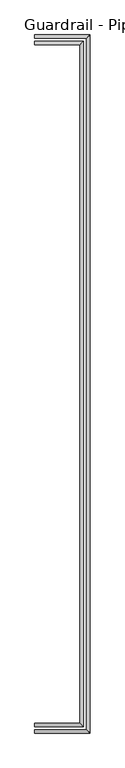
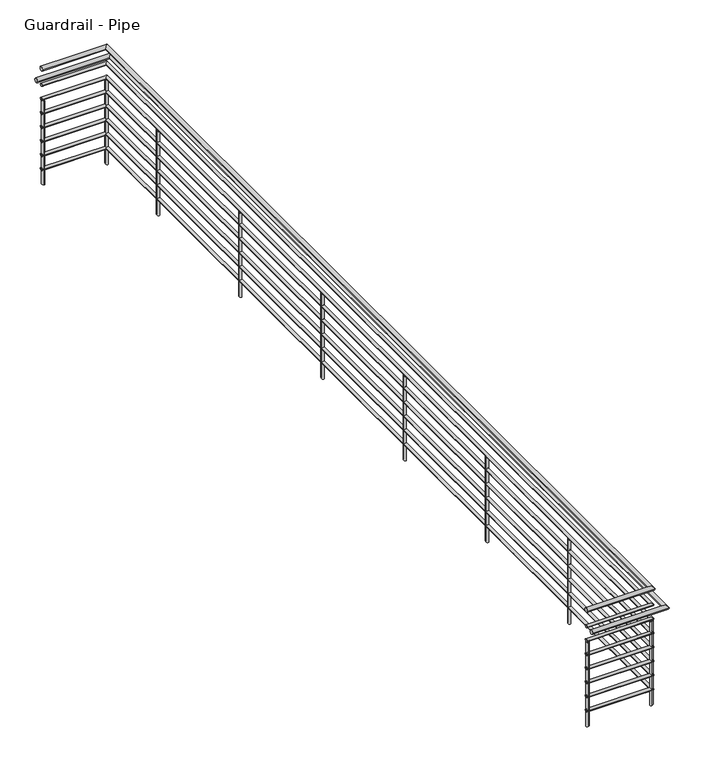
"""IFC4 building model written with IfcOpenShell, lengths in millimetres: railing geometry, Guardrail - Pipe."""

import ifcopenshell
import ifcopenshell.guid

model = None  # the IFC model being written
_history = None  # IfcOwnerHistory: only IFC2X3 demands one
_inside = {}  # id of a spatial element -> (the spatial element, [elements in it])
_under = {}  # id of a project, library or spatial element -> (it, [spatial elements below it])
_declared = {}  # id of a project -> (the project, [libraries it declares])
_typed = {}  # id of a type object -> (the type object, [elements of that type])
_made_of = {}  # id of a material, layer set ... -> (it, [elements and type objects made of it])


def new_model(schema):
    """Start an empty IFC model of exactly this schema.

    Asked for "IFC4X3", IfcOpenShell would pick the latest addendum, in which some entities
    have other attributes; the version numbers below select the first issue.
    IFC2X3 requires an IfcOwnerHistory on every rooted entity: one is made here for all.
    """
    global model, _history
    if schema == "IFC4X3":
        model = ifcopenshell.file(schema_version=(4, 3, 0, 0))
    else:
        model = ifcopenshell.file(schema=schema)
    _inside.clear()
    _under.clear()
    _declared.clear()
    _typed.clear()
    _made_of.clear()
    _history = None
    if model.schema == "IFC2X3":
        org = make("IfcOrganization", Name="unknown")
        user = make(
            "IfcPersonAndOrganization",
            ThePerson=make("IfcPerson", FamilyName="unknown"),
            TheOrganization=org,
        )
        app = make(
            "IfcApplication",
            ApplicationDeveloper=org,
            Version="unknown",
            ApplicationFullName="unknown",
            ApplicationIdentifier="unknown",
        )
        _history = make(
            "IfcOwnerHistory",
            OwningUser=user,
            OwningApplication=app,
            ChangeAction="ADDED",
            CreationDate=0,
        )
    return model


def make(cls, **values):
    """One entity of the class cls with the attributes given. An attribute that is None is left unset."""
    return model.create_entity(
        cls, **{name: value for name, value in values.items() if value is not None}
    )


def rooted(cls, **values):
    """An entity with a GlobalId (a new one), such as an element, a storey or a relation."""
    return make(cls, GlobalId=ifcopenshell.guid.new(), OwnerHistory=_history, **values)


def si_unit(unit_type, name, prefix=None):
    """IfcSIUnit, for example si_unit("LENGTHUNIT", "METRE", prefix="MILLI")."""
    return make("IfcSIUnit", UnitType=unit_type, Prefix=prefix, Name=name)


def assignment(units):
    """IfcUnitAssignment: the units of a project."""
    return None if units is None else make("IfcUnitAssignment", Units=units)


def point(xyz):
    """IfcCartesianPoint."""
    return None if xyz is None else make("IfcCartesianPoint", Coordinates=xyz)


def direction(xyz):
    """IfcDirection."""
    return None if xyz is None else make("IfcDirection", DirectionRatios=xyz)


def frame(location, z_axis=None, x_axis=None):
    """IfcAxis2Placement3D, a coordinate frame: its origin and axes. An axis left out is left unset."""
    return make(
        "IfcAxis2Placement3D",
        Location=point(location),
        Axis=direction(z_axis),
        RefDirection=direction(x_axis),
    )


def origin():
    """The frame at (0, 0, 0) with its axes left unset."""
    return frame((0.0, 0.0, 0.0))


def place(relative_to, where):
    """IfcLocalPlacement: puts the frame where relative to a parent placement (None: the world)."""
    return make(
        "IfcLocalPlacement", PlacementRelTo=relative_to, RelativePlacement=where
    )


def context(
    kind, dimensions, precision=None, world=None, true_north=None, identifier=None
):
    """IfcGeometricRepresentationContext, for example the 3D "Model" context."""
    return make(
        "IfcGeometricRepresentationContext",
        ContextIdentifier=identifier,
        ContextType=kind,
        CoordinateSpaceDimension=dimensions,
        Precision=precision,
        WorldCoordinateSystem=world,
        TrueNorth=true_north,
    )


def project(units=None, contexts=None):
    """IfcProject with its units and contexts."""
    return rooted(
        "IfcProject",
        Name="project",
        RepresentationContexts=contexts,
        UnitsInContext=assignment(units),
    )


def spatial(cls, under=None, at=None, **own):
    """A site, building, storey or space (cls), placed at a placement, below another one or the project."""
    s = rooted(cls, ObjectPlacement=at, **own)
    if under is not None:
        _under.setdefault(under.id(), (under, []))[1].append(s)
    return s


def circle_curve(where, radius):
    """IfcCircle in the frame where."""
    return make("IfcCircle", Position=where, Radius=radius)


def ellipse_curve(where, semi_axis1, semi_axis2):
    """IfcEllipse in the frame where."""
    return make(
        "IfcEllipse", Position=where, SemiAxis1=semi_axis1, SemiAxis2=semi_axis2
    )


def shape(context_of_items, identifier, shape_type, items):
    """IfcShapeRepresentation: the items that make up one representation, for example the "Body"."""
    return make(
        "IfcShapeRepresentation",
        ContextOfItems=context_of_items,
        RepresentationIdentifier=identifier,
        RepresentationType=shape_type,
        Items=items,
    )


def source(mapping_origin, context_of_items, identifier, shape_type, items):
    """IfcRepresentationMap: a shape defined once, which mapped items show again and again."""
    return make(
        "IfcRepresentationMap",
        MappingOrigin=mapping_origin,
        MappedRepresentation=shape(context_of_items, identifier, shape_type, items),
    )


def transform(
    local_origin,
    x_axis=None,
    y_axis=None,
    z_axis=None,
    scale=None,
    scale2=None,
    scale3=None,
    uniform=True,
):
    """IfcCartesianTransformationOperator3D, or its non-uniform kind. x_axis, y_axis, z_axis: its Axis1, 2, 3."""
    if uniform:
        return make(
            "IfcCartesianTransformationOperator3D",
            Axis1=direction(x_axis),
            Axis2=direction(y_axis),
            LocalOrigin=point(local_origin),
            Scale=scale,
            Axis3=direction(z_axis),
        )
    return make(
        "IfcCartesianTransformationOperator3DnonUniform",
        Axis1=direction(x_axis),
        Axis2=direction(y_axis),
        LocalOrigin=point(local_origin),
        Scale=scale,
        Axis3=direction(z_axis),
        Scale2=scale2,
        Scale3=scale3,
    )


def mapped(mapping_source, mapping_target):
    """IfcMappedItem: shows the shape of a source again, moved by a transform."""
    return make(
        "IfcMappedItem", MappingSource=mapping_source, MappingTarget=mapping_target
    )


def made_of(thing, what):
    """Note that an element or type object is made of a material, layer set ...; save() writes the relation."""
    if what is not None:
        _made_of.setdefault(what.id(), (what, []))[1].append(thing)
    return thing


def element(
    cls,
    number,
    at=None,
    inside=None,
    cuts=None,
    type_object=None,
    material=None,
    context=None,
    identifier="Body",
    shape_type=None,
    held_by="IfcProductDefinitionShape",
    body=None,
    shapes=None,
    **own,
):
    """One element of the class cls, such as IfcWall. Its Tag is "e" and its number.

    at: its placement. inside: the storey or other place that contains it. cuts: it is an
    opening in that element (IfcRelVoidsElement). A single representation is given by context,
    identifier, shape_type and body (its items); several are given by shapes. held_by: the class
    of the entity that holds the representations. save() writes the other relations.
    """
    e = rooted(cls, Tag="e%d" % number, ObjectPlacement=at, **own)
    if body is not None:
        shapes = [shape(context, identifier, shape_type, body)]
    if shapes is not None:
        e.Representation = make(held_by, Representations=shapes)
    if inside is not None:
        _inside.setdefault(inside.id(), (inside, []))[1].append(e)
    if cuts is not None:
        rooted(
            "IfcRelVoidsElement", RelatingBuildingElement=cuts, RelatedOpeningElement=e
        )
    if type_object is not None:
        _typed.setdefault(type_object.id(), (type_object, []))[1].append(e)
    return made_of(e, material)


def aggregate(whole, parts):
    """IfcRelAggregates: a whole, such as a stair, and the parts it consists of."""
    return rooted("IfcRelAggregates", RelatingObject=whole, RelatedObjects=parts)


def save(model, path):
    """Write the relations noted so far, then the file.

    IfcRelAggregates (storeys below a building ...), IfcRelContainedInSpatialStructure (elements
    in a storey), IfcRelDefinesByType, IfcRelAssociatesMaterial and IfcRelDeclares: one each for
    every whole, place, type object, material and project.
    """
    for whole, parts in _under.values():
        aggregate(whole, parts)
    for where, things in _inside.values():
        rooted(
            "IfcRelContainedInSpatialStructure",
            RelatedElements=things,
            RelatingStructure=where,
        )
    for kind, things in _typed.values():
        rooted("IfcRelDefinesByType", RelatedObjects=things, RelatingType=kind)
    for what, things in _made_of.values():
        rooted("IfcRelAssociatesMaterial", RelatedObjects=things, RelatingMaterial=what)
    for by, libraries in _declared.values():
        rooted("IfcRelDeclares", RelatingContext=by, RelatedDefinitions=libraries)
    model.write(path)


def plane_surface(at):
    """IfcPlane: the flat surface through the origin of the frame at, square to its z axis."""
    return make("IfcPlane", Position=at)


def cylinder_surface(at, radius):
    """IfcCylindricalSurface: all points at the distance radius from the z axis of the frame at."""
    return make("IfcCylindricalSurface", Position=at, Radius=radius)


def advanced_brep(points, edges, surfaces, faces):
    """IfcAdvancedBrep: a solid bounded by faces that lie on surfaces and meet in shared edges.

    An edge is (start, end): straight between two places in points (the first is 0);
    or (start, end, curve); or (start, end, curve, False) where it runs against its curve.
    A face is (place in surfaces, loops), or (place, loops, False) where it looks against
    its surface's normal. A loop lists edges by number (the first is 1), with a minus sign
    where the edge is run from its end to its start. The first loop is the outer one.
    """
    corners = [point(p) for p in points]
    vertices = [make("IfcVertexPoint", VertexGeometry=c) for c in corners]
    made = []
    for start, end, *more in edges:
        made.append(
            make(
                "IfcEdgeCurve",
                EdgeStart=vertices[start],
                EdgeEnd=vertices[end],
                EdgeGeometry=more[0] if more else make("IfcPolyline", Points=[corners[start], corners[end]]),
                SameSense=more[1] if len(more) > 1 else True,
            )
        )
    hull = []
    for where, loops, *sense in faces:
        bounds = []
        for j, loop in enumerate(loops):
            ring = [make("IfcOrientedEdge", EdgeElement=made[abs(k) - 1], Orientation=k > 0) for k in loop]
            bounds.append(
                make(
                    "IfcFaceOuterBound" if j == 0 else "IfcFaceBound",
                    Bound=make("IfcEdgeLoop", EdgeList=ring),
                    Orientation=True,
                )
            )
        hull.append(make("IfcAdvancedFace", Bounds=bounds, FaceSurface=surfaces[where], SameSense=sense[0] if sense else True))
    return make("IfcAdvancedBrep", Outer=make("IfcClosedShell", CfsFaces=hull))


def guardrail_pipe_ba8d120a(model_context):
    return source(origin(), model_context, "Body", "AdvancedBrep", [
        advanced_brep(
        [(13389.3313551, 10867.95, 4705.35), (13389.3313551, 10906.05, 4705.35), (13967.1813551, 10867.95, 4705.35), (13929.0813551, 10906.05, 4705.35), (13967.1813551, 18983.25, 4705.35), (13929.0813551, 18945.15, 4705.35), (13389.3313551, 18983.25, 4705.35), (13389.3313551, 18945.15, 4705.35)],
        [
            (0, 1, circle_curve(frame((13389.3313551, 10887.0, 4705.35), z_axis=(-1.0, 0.0, 0.0), x_axis=(0.0, 1.0, 0.0)), 19.05)),
            (1, 0, circle_curve(frame((13389.3313551, 10887.0, 4705.35), z_axis=(-1.0, 0.0, 0.0), x_axis=(0.0, 1.0, 0.0)), 19.05)),
            (0, 2),
            (2, 3, ellipse_curve(frame((13948.1313551, 10887.0, 4705.35), z_axis=(-0.7071067811865475, -0.7071067811865475, 0.0), x_axis=(-0.7071067811865476, 0.7071067811865474, 0.0)), 26.9407684, 19.05)),
            (3, 1),
            (3, 2, ellipse_curve(frame((13948.1313551, 10887.0, 4705.35), z_axis=(-0.7071067811865475, -0.7071067811865475, 0.0), x_axis=(-0.7071067811865476, 0.7071067811865474, 0.0)), 26.9407684, 19.05)),
            (2, 4),
            (4, 5, ellipse_curve(frame((13948.1313551, 18964.2, 4705.35), z_axis=(0.7071067811865475, -0.7071067811865475, 0.0), x_axis=(-0.7071067811865474, -0.7071067811865476, 0.0)), 26.9407684, 19.05)),
            (5, 3),
            (5, 4, ellipse_curve(frame((13948.1313551, 18964.2, 4705.35), z_axis=(0.7071067811865475, -0.7071067811865475, 0.0), x_axis=(-0.7071067811865474, -0.7071067811865476, 0.0)), 26.9407684, 19.05)),
            (6, 7, circle_curve(frame((13389.3313551, 18964.2, 4705.35), z_axis=(-1.0, 0.0, 0.0), x_axis=(0.0, -1.0, 0.0)), 19.05)),
            (7, 6, circle_curve(frame((13389.3313551, 18964.2, 4705.35), z_axis=(-1.0, 0.0, 0.0), x_axis=(0.0, -1.0, 0.0)), 19.05)),
            (4, 6),
            (7, 5),
        ],
        [
            plane_surface(frame((13389.3313551, 10887.0, 4724.4), z_axis=(-1.0, 0.0, 0.0), x_axis=(0.0, 1.0, 0.0))),
            cylinder_surface(frame((13389.3313551, 10887.0, 4705.35), z_axis=(-1.0, 0.0, 0.0), x_axis=(0.0, 1.0, 0.0)), 19.05),
            cylinder_surface(frame((13948.1313551, 10887.0, 4705.35), z_axis=(0.0, -1.0, 0.0), x_axis=(-1.0, 0.0, 0.0)), 19.05),
            plane_surface(frame((13389.3313551, 18964.2, 4724.4), z_axis=(-1.0, 0.0, 0.0), x_axis=(0.0, -1.0, 0.0))),
            cylinder_surface(frame((13948.1313551, 18964.2, 4705.35), z_axis=(1.0, 0.0, 0.0), x_axis=(0.0, -1.0, 0.0)), 19.05),
        ],
        [
            (0, [[1, 2]]),
            (1, [[-1, 3, 4, 5]]),
            (1, [[-2, -5, 6, -3]]),
            (2, [[-4, 7, 8, 9]]),
            (2, [[-6, -9, 10, -7]]),
            (3, [[11, 12]]),
            (4, [[-8, 13, -12, 14]]),
            (4, [[-10, -14, -11, -13]]),
        ],
    ),
        advanced_brep(
        [(13389.3313551, 10874.3, 4559.3), (13389.3313551, 10899.7, 4559.3), (13960.8313551, 10874.3, 4559.3), (13935.4313551, 10899.7, 4559.3), (13960.8313551, 18976.9, 4559.3), (13935.4313551, 18951.5, 4559.3), (13389.3313551, 18976.9, 4559.3), (13389.3313551, 18951.5, 4559.3)],
        [
            (0, 1, circle_curve(frame((13389.3313551, 10887.0, 4559.3), z_axis=(-1.0, 0.0, 0.0), x_axis=(0.0, 1.0, 0.0)), 12.7)),
            (1, 0, circle_curve(frame((13389.3313551, 10887.0, 4559.3), z_axis=(-1.0, 0.0, 0.0), x_axis=(0.0, 1.0, 0.0)), 12.7)),
            (0, 2),
            (2, 3, ellipse_curve(frame((13948.1313551, 10887.0, 4559.3), z_axis=(-0.7071067811865475, -0.7071067811865475, 0.0), x_axis=(-0.7071067811865476, 0.7071067811865474, 0.0)), 17.9605122, 12.7)),
            (3, 1),
            (3, 2, ellipse_curve(frame((13948.1313551, 10887.0, 4559.3), z_axis=(-0.7071067811865475, -0.7071067811865475, 0.0), x_axis=(-0.7071067811865476, 0.7071067811865474, 0.0)), 17.9605122, 12.7)),
            (2, 4),
            (4, 5, ellipse_curve(frame((13948.1313551, 18964.2, 4559.3), z_axis=(0.7071067811865475, -0.7071067811865475, 0.0), x_axis=(-0.7071067811865474, -0.7071067811865476, 0.0)), 17.9605122, 12.7)),
            (5, 3),
            (5, 4, ellipse_curve(frame((13948.1313551, 18964.2, 4559.3), z_axis=(0.7071067811865475, -0.7071067811865475, 0.0), x_axis=(-0.7071067811865474, -0.7071067811865476, 0.0)), 17.9605122, 12.7)),
            (6, 7, circle_curve(frame((13389.3313551, 18964.2, 4559.3), z_axis=(-1.0, 0.0, 0.0), x_axis=(0.0, -1.0, 0.0)), 12.7)),
            (7, 6, circle_curve(frame((13389.3313551, 18964.2, 4559.3), z_axis=(-1.0, 0.0, 0.0), x_axis=(0.0, -1.0, 0.0)), 12.7)),
            (4, 6),
            (7, 5),
        ],
        [
            plane_surface(frame((13389.3313551, 10887.0, 4572.0), z_axis=(-1.0, 0.0, 0.0), x_axis=(0.0, 1.0, 0.0))),
            cylinder_surface(frame((13389.3313551, 10887.0, 4559.3), z_axis=(-1.0, 0.0, 0.0), x_axis=(0.0, 1.0, 0.0)), 12.7),
            cylinder_surface(frame((13948.1313551, 10887.0, 4559.3), z_axis=(0.0, -1.0, 0.0), x_axis=(-1.0, 0.0, 0.0)), 12.7),
            plane_surface(frame((13389.3313551, 18964.2, 4572.0), z_axis=(-1.0, 0.0, 0.0), x_axis=(0.0, -1.0, 0.0))),
            cylinder_surface(frame((13948.1313551, 18964.2, 4559.3), z_axis=(1.0, 0.0, 0.0), x_axis=(0.0, -1.0, 0.0)), 12.7),
        ],
        [
            (0, [[1, 2]]),
            (1, [[-1, 3, 4, 5]]),
            (1, [[-2, -5, 6, -3]]),
            (2, [[-4, 7, 8, 9]]),
            (2, [[-6, -9, 10, -7]]),
            (3, [[11, 12]]),
            (4, [[-8, 13, -12, 14]]),
            (4, [[-10, -14, -11, -13]]),
        ],
    ),
        advanced_brep(
        [(13389.3313551, 10791.75, 4552.95), (13389.3313551, 10829.85, 4552.95), (14043.3813551, 10791.75, 4552.95), (14005.2813551, 10829.85, 4552.95), (14043.3813551, 19059.45, 4552.95), (14005.2813551, 19021.35, 4552.95), (13389.3313551, 19059.45, 4552.95), (13389.3313551, 19021.35, 4552.95)],
        [
            (0, 1, circle_curve(frame((13389.3313551, 10810.8, 4552.95), z_axis=(-1.0, 0.0, 0.0), x_axis=(0.0, 1.0, 0.0)), 19.05)),
            (1, 0, circle_curve(frame((13389.3313551, 10810.8, 4552.95), z_axis=(-1.0, 0.0, 0.0), x_axis=(0.0, 1.0, 0.0)), 19.05)),
            (0, 2),
            (2, 3, ellipse_curve(frame((14024.3313551, 10810.8, 4552.95), z_axis=(-0.7071067811865475, -0.7071067811865475, 0.0), x_axis=(-0.7071067811865476, 0.7071067811865474, 0.0)), 26.9407684, 19.05)),
            (3, 1),
            (3, 2, ellipse_curve(frame((14024.3313551, 10810.8, 4552.95), z_axis=(-0.7071067811865475, -0.7071067811865475, 0.0), x_axis=(-0.7071067811865476, 0.7071067811865474, 0.0)), 26.9407684, 19.05)),
            (2, 4),
            (4, 5, ellipse_curve(frame((14024.3313551, 19040.4, 4552.95), z_axis=(0.7071067811865475, -0.7071067811865475, 0.0), x_axis=(-0.7071067811865474, -0.7071067811865476, 0.0)), 26.9407684, 19.05)),
            (5, 3),
            (5, 4, ellipse_curve(frame((14024.3313551, 19040.4, 4552.95), z_axis=(0.7071067811865475, -0.7071067811865475, 0.0), x_axis=(-0.7071067811865474, -0.7071067811865476, 0.0)), 26.9407684, 19.05)),
            (6, 7, circle_curve(frame((13389.3313551, 19040.4, 4552.95), z_axis=(-1.0, 0.0, 0.0), x_axis=(0.0, -1.0, 0.0)), 19.05)),
            (7, 6, circle_curve(frame((13389.3313551, 19040.4, 4552.95), z_axis=(-1.0, 0.0, 0.0), x_axis=(0.0, -1.0, 0.0)), 19.05)),
            (4, 6),
            (7, 5),
        ],
        [
            plane_surface(frame((13389.3313551, 10810.8, 4572.0), z_axis=(-1.0, 0.0, 0.0), x_axis=(0.0, 1.0, 0.0))),
            cylinder_surface(frame((13389.3313551, 10810.8, 4552.95), z_axis=(-1.0, 0.0, 0.0), x_axis=(0.0, 1.0, 0.0)), 19.05),
            cylinder_surface(frame((14024.3313551, 10810.8, 4552.95), z_axis=(0.0, -1.0, 0.0), x_axis=(-1.0, 0.0, 0.0)), 19.05),
            plane_surface(frame((13389.3313551, 19040.4, 4572.0), z_axis=(-1.0, 0.0, 0.0), x_axis=(0.0, -1.0, 0.0))),
            cylinder_surface(frame((14024.3313551, 19040.4, 4552.95), z_axis=(1.0, 0.0, 0.0), x_axis=(0.0, -1.0, 0.0)), 19.05),
        ],
        [
            (0, [[1, 2]]),
            (1, [[-1, 3, 4, 5]]),
            (1, [[-2, -5, 6, -3]]),
            (2, [[-4, 7, 8, 9]]),
            (2, [[-6, -9, 10, -7]]),
            (3, [[11, 12]]),
            (4, [[-8, 13, -12, 14]]),
            (4, [[-10, -14, -11, -13]]),
        ],
    ),
        advanced_brep(
        [(13389.3313551, 10874.3, 4432.3), (13389.3313551, 10899.7, 4432.3), (13960.8313551, 10874.3, 4432.3), (13935.4313551, 10899.7, 4432.3), (13960.8313551, 18976.9, 4432.3), (13935.4313551, 18951.5, 4432.3), (13389.3313551, 18976.9, 4432.3), (13389.3313551, 18951.5, 4432.3)],
        [
            (0, 1, circle_curve(frame((13389.3313551, 10887.0, 4432.3), z_axis=(-1.0, 0.0, 0.0), x_axis=(0.0, 1.0, 0.0)), 12.7)),
            (1, 0, circle_curve(frame((13389.3313551, 10887.0, 4432.3), z_axis=(-1.0, 0.0, 0.0), x_axis=(0.0, 1.0, 0.0)), 12.7)),
            (0, 2),
            (2, 3, ellipse_curve(frame((13948.1313551, 10887.0, 4432.3), z_axis=(-0.7071067811865475, -0.7071067811865475, 0.0), x_axis=(-0.7071067811865476, 0.7071067811865474, 0.0)), 17.9605122, 12.7)),
            (3, 1),
            (3, 2, ellipse_curve(frame((13948.1313551, 10887.0, 4432.3), z_axis=(-0.7071067811865475, -0.7071067811865475, 0.0), x_axis=(-0.7071067811865476, 0.7071067811865474, 0.0)), 17.9605122, 12.7)),
            (2, 4),
            (4, 5, ellipse_curve(frame((13948.1313551, 18964.2, 4432.3), z_axis=(0.7071067811865475, -0.7071067811865475, 0.0), x_axis=(-0.7071067811865474, -0.7071067811865476, 0.0)), 17.9605122, 12.7)),
            (5, 3),
            (5, 4, ellipse_curve(frame((13948.1313551, 18964.2, 4432.3), z_axis=(0.7071067811865475, -0.7071067811865475, 0.0), x_axis=(-0.7071067811865474, -0.7071067811865476, 0.0)), 17.9605122, 12.7)),
            (6, 7, circle_curve(frame((13389.3313551, 18964.2, 4432.3), z_axis=(-1.0, 0.0, 0.0), x_axis=(0.0, -1.0, 0.0)), 12.7)),
            (7, 6, circle_curve(frame((13389.3313551, 18964.2, 4432.3), z_axis=(-1.0, 0.0, 0.0), x_axis=(0.0, -1.0, 0.0)), 12.7)),
            (4, 6),
            (7, 5),
        ],
        [
            plane_surface(frame((13389.3313551, 10887.0, 4445.0), z_axis=(-1.0, 0.0, 0.0), x_axis=(0.0, 1.0, 0.0))),
            cylinder_surface(frame((13389.3313551, 10887.0, 4432.3), z_axis=(-1.0, 0.0, 0.0), x_axis=(0.0, 1.0, 0.0)), 12.7),
            cylinder_surface(frame((13948.1313551, 10887.0, 4432.3), z_axis=(0.0, -1.0, 0.0), x_axis=(-1.0, 0.0, 0.0)), 12.7),
            plane_surface(frame((13389.3313551, 18964.2, 4445.0), z_axis=(-1.0, 0.0, 0.0), x_axis=(0.0, -1.0, 0.0))),
            cylinder_surface(frame((13948.1313551, 18964.2, 4432.3), z_axis=(1.0, 0.0, 0.0), x_axis=(0.0, -1.0, 0.0)), 12.7),
        ],
        [
            (0, [[1, 2]]),
            (1, [[-1, 3, 4, 5]]),
            (1, [[-2, -5, 6, -3]]),
            (2, [[-4, 7, 8, 9]]),
            (2, [[-6, -9, 10, -7]]),
            (3, [[11, 12]]),
            (4, [[-8, 13, -12, 14]]),
            (4, [[-10, -14, -11, -13]]),
        ],
    ),
        advanced_brep(
        [(13389.3313551, 10874.3, 4305.3), (13389.3313551, 10899.7, 4305.3), (13960.8313551, 10874.3, 4305.3), (13935.4313551, 10899.7, 4305.3), (13960.8313551, 18976.9, 4305.3), (13935.4313551, 18951.5, 4305.3), (13389.3313551, 18976.9, 4305.3), (13389.3313551, 18951.5, 4305.3)],
        [
            (0, 1, circle_curve(frame((13389.3313551, 10887.0, 4305.3), z_axis=(-1.0, 0.0, 0.0), x_axis=(0.0, 1.0, 0.0)), 12.7)),
            (1, 0, circle_curve(frame((13389.3313551, 10887.0, 4305.3), z_axis=(-1.0, 0.0, 0.0), x_axis=(0.0, 1.0, 0.0)), 12.7)),
            (0, 2),
            (2, 3, ellipse_curve(frame((13948.1313551, 10887.0, 4305.3), z_axis=(-0.7071067811865475, -0.7071067811865475, 0.0), x_axis=(-0.7071067811865476, 0.7071067811865474, 0.0)), 17.9605122, 12.7)),
            (3, 1),
            (3, 2, ellipse_curve(frame((13948.1313551, 10887.0, 4305.3), z_axis=(-0.7071067811865475, -0.7071067811865475, 0.0), x_axis=(-0.7071067811865476, 0.7071067811865474, 0.0)), 17.9605122, 12.7)),
            (2, 4),
            (4, 5, ellipse_curve(frame((13948.1313551, 18964.2, 4305.3), z_axis=(0.7071067811865475, -0.7071067811865475, 0.0), x_axis=(-0.7071067811865474, -0.7071067811865476, 0.0)), 17.9605122, 12.7)),
            (5, 3),
            (5, 4, ellipse_curve(frame((13948.1313551, 18964.2, 4305.3), z_axis=(0.7071067811865475, -0.7071067811865475, 0.0), x_axis=(-0.7071067811865474, -0.7071067811865476, 0.0)), 17.9605122, 12.7)),
            (6, 7, circle_curve(frame((13389.3313551, 18964.2, 4305.3), z_axis=(-1.0, 0.0, 0.0), x_axis=(0.0, -1.0, 0.0)), 12.7)),
            (7, 6, circle_curve(frame((13389.3313551, 18964.2, 4305.3), z_axis=(-1.0, 0.0, 0.0), x_axis=(0.0, -1.0, 0.0)), 12.7)),
            (4, 6),
            (7, 5),
        ],
        [
            plane_surface(frame((13389.3313551, 10887.0, 4318.0), z_axis=(-1.0, 0.0, 0.0), x_axis=(0.0, 1.0, 0.0))),
            cylinder_surface(frame((13389.3313551, 10887.0, 4305.3), z_axis=(-1.0, 0.0, 0.0), x_axis=(0.0, 1.0, 0.0)), 12.7),
            cylinder_surface(frame((13948.1313551, 10887.0, 4305.3), z_axis=(0.0, -1.0, 0.0), x_axis=(-1.0, 0.0, 0.0)), 12.7),
            plane_surface(frame((13389.3313551, 18964.2, 4318.0), z_axis=(-1.0, 0.0, 0.0), x_axis=(0.0, -1.0, 0.0))),
            cylinder_surface(frame((13948.1313551, 18964.2, 4305.3), z_axis=(1.0, 0.0, 0.0), x_axis=(0.0, -1.0, 0.0)), 12.7),
        ],
        [
            (0, [[1, 2]]),
            (1, [[-1, 3, 4, 5]]),
            (1, [[-2, -5, 6, -3]]),
            (2, [[-4, 7, 8, 9]]),
            (2, [[-6, -9, 10, -7]]),
            (3, [[11, 12]]),
            (4, [[-8, 13, -12, 14]]),
            (4, [[-10, -14, -11, -13]]),
        ],
    ),
        advanced_brep(
        [(13389.3313551, 10874.3, 4178.3), (13389.3313551, 10899.7, 4178.3), (13960.8313551, 10874.3, 4178.3), (13935.4313551, 10899.7, 4178.3), (13960.8313551, 18976.9, 4178.3), (13935.4313551, 18951.5, 4178.3), (13389.3313551, 18976.9, 4178.3), (13389.3313551, 18951.5, 4178.3)],
        [
            (0, 1, circle_curve(frame((13389.3313551, 10887.0, 4178.3), z_axis=(-1.0, 0.0, 0.0), x_axis=(0.0, 1.0, 0.0)), 12.7)),
            (1, 0, circle_curve(frame((13389.3313551, 10887.0, 4178.3), z_axis=(-1.0, 0.0, 0.0), x_axis=(0.0, 1.0, 0.0)), 12.7)),
            (0, 2),
            (2, 3, ellipse_curve(frame((13948.1313551, 10887.0, 4178.3), z_axis=(-0.7071067811865475, -0.7071067811865475, 0.0), x_axis=(-0.7071067811865476, 0.7071067811865474, 0.0)), 17.9605122, 12.7)),
            (3, 1),
            (3, 2, ellipse_curve(frame((13948.1313551, 10887.0, 4178.3), z_axis=(-0.7071067811865475, -0.7071067811865475, 0.0), x_axis=(-0.7071067811865476, 0.7071067811865474, 0.0)), 17.9605122, 12.7)),
            (2, 4),
            (4, 5, ellipse_curve(frame((13948.1313551, 18964.2, 4178.3), z_axis=(0.7071067811865475, -0.7071067811865475, 0.0), x_axis=(-0.7071067811865474, -0.7071067811865476, 0.0)), 17.9605122, 12.7)),
            (5, 3),
            (5, 4, ellipse_curve(frame((13948.1313551, 18964.2, 4178.3), z_axis=(0.7071067811865475, -0.7071067811865475, 0.0), x_axis=(-0.7071067811865474, -0.7071067811865476, 0.0)), 17.9605122, 12.7)),
            (6, 7, circle_curve(frame((13389.3313551, 18964.2, 4178.3), z_axis=(-1.0, 0.0, 0.0), x_axis=(0.0, -1.0, 0.0)), 12.7)),
            (7, 6, circle_curve(frame((13389.3313551, 18964.2, 4178.3), z_axis=(-1.0, 0.0, 0.0), x_axis=(0.0, -1.0, 0.0)), 12.7)),
            (4, 6),
            (7, 5),
        ],
        [
            plane_surface(frame((13389.3313551, 10887.0, 4191.0), z_axis=(-1.0, 0.0, 0.0), x_axis=(0.0, 1.0, 0.0))),
            cylinder_surface(frame((13389.3313551, 10887.0, 4178.3), z_axis=(-1.0, 0.0, 0.0), x_axis=(0.0, 1.0, 0.0)), 12.7),
            cylinder_surface(frame((13948.1313551, 10887.0, 4178.3), z_axis=(0.0, -1.0, 0.0), x_axis=(-1.0, 0.0, 0.0)), 12.7),
            plane_surface(frame((13389.3313551, 18964.2, 4191.0), z_axis=(-1.0, 0.0, 0.0), x_axis=(0.0, -1.0, 0.0))),
            cylinder_surface(frame((13948.1313551, 18964.2, 4178.3), z_axis=(1.0, 0.0, 0.0), x_axis=(0.0, -1.0, 0.0)), 12.7),
        ],
        [
            (0, [[1, 2]]),
            (1, [[-1, 3, 4, 5]]),
            (1, [[-2, -5, 6, -3]]),
            (2, [[-4, 7, 8, 9]]),
            (2, [[-6, -9, 10, -7]]),
            (3, [[11, 12]]),
            (4, [[-8, 13, -12, 14]]),
            (4, [[-10, -14, -11, -13]]),
        ],
    ),
        advanced_brep(
        [(13389.3313551, 10874.3, 4051.3), (13389.3313551, 10899.7, 4051.3), (13960.8313551, 10874.3, 4051.3), (13935.4313551, 10899.7, 4051.3), (13960.8313551, 18976.9, 4051.3), (13935.4313551, 18951.5, 4051.3), (13389.3313551, 18976.9, 4051.3), (13389.3313551, 18951.5, 4051.3)],
        [
            (0, 1, circle_curve(frame((13389.3313551, 10887.0, 4051.3), z_axis=(-1.0, 0.0, 0.0), x_axis=(0.0, 1.0, 0.0)), 12.7)),
            (1, 0, circle_curve(frame((13389.3313551, 10887.0, 4051.3), z_axis=(-1.0, 0.0, 0.0), x_axis=(0.0, 1.0, 0.0)), 12.7)),
            (0, 2),
            (2, 3, ellipse_curve(frame((13948.1313551, 10887.0, 4051.3), z_axis=(-0.7071067811865475, -0.7071067811865475, 0.0), x_axis=(-0.7071067811865476, 0.7071067811865474, 0.0)), 17.9605122, 12.7)),
            (3, 1),
            (3, 2, ellipse_curve(frame((13948.1313551, 10887.0, 4051.3), z_axis=(-0.7071067811865475, -0.7071067811865475, 0.0), x_axis=(-0.7071067811865476, 0.7071067811865474, 0.0)), 17.9605122, 12.7)),
            (2, 4),
            (4, 5, ellipse_curve(frame((13948.1313551, 18964.2, 4051.3), z_axis=(0.7071067811865475, -0.7071067811865475, 0.0), x_axis=(-0.7071067811865474, -0.7071067811865476, 0.0)), 17.9605122, 12.7)),
            (5, 3),
            (5, 4, ellipse_curve(frame((13948.1313551, 18964.2, 4051.3), z_axis=(0.7071067811865475, -0.7071067811865475, 0.0), x_axis=(-0.7071067811865474, -0.7071067811865476, 0.0)), 17.9605122, 12.7)),
            (6, 7, circle_curve(frame((13389.3313551, 18964.2, 4051.3), z_axis=(-1.0, 0.0, 0.0), x_axis=(0.0, -1.0, 0.0)), 12.7)),
            (7, 6, circle_curve(frame((13389.3313551, 18964.2, 4051.3), z_axis=(-1.0, 0.0, 0.0), x_axis=(0.0, -1.0, 0.0)), 12.7)),
            (4, 6),
            (7, 5),
        ],
        [
            plane_surface(frame((13389.3313551, 10887.0, 4064.0), z_axis=(-1.0, 0.0, 0.0), x_axis=(0.0, 1.0, 0.0))),
            cylinder_surface(frame((13389.3313551, 10887.0, 4051.3), z_axis=(-1.0, 0.0, 0.0), x_axis=(0.0, 1.0, 0.0)), 12.7),
            cylinder_surface(frame((13948.1313551, 10887.0, 4051.3), z_axis=(0.0, -1.0, 0.0), x_axis=(-1.0, 0.0, 0.0)), 12.7),
            plane_surface(frame((13389.3313551, 18964.2, 4064.0), z_axis=(-1.0, 0.0, 0.0), x_axis=(0.0, -1.0, 0.0))),
            cylinder_surface(frame((13948.1313551, 18964.2, 4051.3), z_axis=(1.0, 0.0, 0.0), x_axis=(0.0, -1.0, 0.0)), 12.7),
        ],
        [
            (0, [[1, 2]]),
            (1, [[-1, 3, 4, 5]]),
            (1, [[-2, -5, 6, -3]]),
            (2, [[-4, 7, 8, 9]]),
            (2, [[-6, -9, 10, -7]]),
            (3, [[11, 12]]),
            (4, [[-8, 13, -12, 14]]),
            (4, [[-10, -14, -11, -13]]),
        ],
    ),
        advanced_brep(
        [(13389.3313551, 10874.3, 3924.3), (13389.3313551, 10899.7, 3924.3), (13960.8313551, 10874.3, 3924.3), (13935.4313551, 10899.7, 3924.3), (13960.8313551, 18976.9, 3924.3), (13935.4313551, 18951.5, 3924.3), (13389.3313551, 18976.9, 3924.3), (13389.3313551, 18951.5, 3924.3)],
        [
            (0, 1, circle_curve(frame((13389.3313551, 10887.0, 3924.3), z_axis=(-1.0, 0.0, 0.0), x_axis=(0.0, 1.0, 0.0)), 12.7)),
            (1, 0, circle_curve(frame((13389.3313551, 10887.0, 3924.3), z_axis=(-1.0, 0.0, 0.0), x_axis=(0.0, 1.0, 0.0)), 12.7)),
            (0, 2),
            (2, 3, ellipse_curve(frame((13948.1313551, 10887.0, 3924.3), z_axis=(-0.7071067811865475, -0.7071067811865475, 0.0), x_axis=(-0.7071067811865476, 0.7071067811865474, 0.0)), 17.9605122, 12.7)),
            (3, 1),
            (3, 2, ellipse_curve(frame((13948.1313551, 10887.0, 3924.3), z_axis=(-0.7071067811865475, -0.7071067811865475, 0.0), x_axis=(-0.7071067811865476, 0.7071067811865474, 0.0)), 17.9605122, 12.7)),
            (2, 4),
            (4, 5, ellipse_curve(frame((13948.1313551, 18964.2, 3924.3), z_axis=(0.7071067811865475, -0.7071067811865475, 0.0), x_axis=(-0.7071067811865474, -0.7071067811865476, 0.0)), 17.9605122, 12.7)),
            (5, 3),
            (5, 4, ellipse_curve(frame((13948.1313551, 18964.2, 3924.3), z_axis=(0.7071067811865475, -0.7071067811865475, 0.0), x_axis=(-0.7071067811865474, -0.7071067811865476, 0.0)), 17.9605122, 12.7)),
            (6, 7, circle_curve(frame((13389.3313551, 18964.2, 3924.3), z_axis=(-1.0, 0.0, 0.0), x_axis=(0.0, -1.0, 0.0)), 12.7)),
            (7, 6, circle_curve(frame((13389.3313551, 18964.2, 3924.3), z_axis=(-1.0, 0.0, 0.0), x_axis=(0.0, -1.0, 0.0)), 12.7)),
            (4, 6),
            (7, 5),
        ],
        [
            plane_surface(frame((13389.3313551, 10887.0, 3937.0), z_axis=(-1.0, 0.0, 0.0), x_axis=(0.0, 1.0, 0.0))),
            cylinder_surface(frame((13389.3313551, 10887.0, 3924.3), z_axis=(-1.0, 0.0, 0.0), x_axis=(0.0, 1.0, 0.0)), 12.7),
            cylinder_surface(frame((13948.1313551, 10887.0, 3924.3), z_axis=(0.0, -1.0, 0.0), x_axis=(-1.0, 0.0, 0.0)), 12.7),
            plane_surface(frame((13389.3313551, 18964.2, 3937.0), z_axis=(-1.0, 0.0, 0.0), x_axis=(0.0, -1.0, 0.0))),
            cylinder_surface(frame((13948.1313551, 18964.2, 3924.3), z_axis=(1.0, 0.0, 0.0), x_axis=(0.0, -1.0, 0.0)), 12.7),
        ],
        [
            (0, [[1, 2]]),
            (1, [[-1, 3, 4, 5]]),
            (1, [[-2, -5, 6, -3]]),
            (2, [[-4, 7, 8, 9]]),
            (2, [[-6, -9, 10, -7]]),
            (3, [[11, 12]]),
            (4, [[-8, 13, -12, 14]]),
            (4, [[-10, -14, -11, -13]]),
        ],
    ),
        advanced_brep(
        [(13389.3313551, 10874.3, 3797.3), (13389.3313551, 10899.7, 3797.3), (13960.8313551, 10874.3, 3797.3), (13935.4313551, 10899.7, 3797.3), (13960.8313551, 18976.9, 3797.3), (13935.4313551, 18951.5, 3797.3), (13389.3313551, 18976.9, 3797.3), (13389.3313551, 18951.5, 3797.3)],
        [
            (0, 1, circle_curve(frame((13389.3313551, 10887.0, 3797.3), z_axis=(-1.0, 0.0, 0.0), x_axis=(0.0, 1.0, 0.0)), 12.7)),
            (1, 0, circle_curve(frame((13389.3313551, 10887.0, 3797.3), z_axis=(-1.0, 0.0, 0.0), x_axis=(0.0, 1.0, 0.0)), 12.7)),
            (0, 2),
            (2, 3, ellipse_curve(frame((13948.1313551, 10887.0, 3797.3), z_axis=(-0.7071067811865475, -0.7071067811865475, 0.0), x_axis=(-0.7071067811865476, 0.7071067811865474, 0.0)), 17.9605122, 12.7)),
            (3, 1),
            (3, 2, ellipse_curve(frame((13948.1313551, 10887.0, 3797.3), z_axis=(-0.7071067811865475, -0.7071067811865475, 0.0), x_axis=(-0.7071067811865476, 0.7071067811865474, 0.0)), 17.9605122, 12.7)),
            (2, 4),
            (4, 5, ellipse_curve(frame((13948.1313551, 18964.2, 3797.3), z_axis=(0.7071067811865475, -0.7071067811865475, 0.0), x_axis=(-0.7071067811865474, -0.7071067811865476, 0.0)), 17.9605122, 12.7)),
            (5, 3),
            (5, 4, ellipse_curve(frame((13948.1313551, 18964.2, 3797.3), z_axis=(0.7071067811865475, -0.7071067811865475, 0.0), x_axis=(-0.7071067811865474, -0.7071067811865476, 0.0)), 17.9605122, 12.7)),
            (6, 7, circle_curve(frame((13389.3313551, 18964.2, 3797.3), z_axis=(-1.0, 0.0, 0.0), x_axis=(0.0, -1.0, 0.0)), 12.7)),
            (7, 6, circle_curve(frame((13389.3313551, 18964.2, 3797.3), z_axis=(-1.0, 0.0, 0.0), x_axis=(0.0, -1.0, 0.0)), 12.7)),
            (4, 6),
            (7, 5),
        ],
        [
            plane_surface(frame((13389.3313551, 10887.0, 3810.0), z_axis=(-1.0, 0.0, 0.0), x_axis=(0.0, 1.0, 0.0))),
            cylinder_surface(frame((13389.3313551, 10887.0, 3797.3), z_axis=(-1.0, 0.0, 0.0), x_axis=(0.0, 1.0, 0.0)), 12.7),
            cylinder_surface(frame((13948.1313551, 10887.0, 3797.3), z_axis=(0.0, -1.0, 0.0), x_axis=(-1.0, 0.0, 0.0)), 12.7),
            plane_surface(frame((13389.3313551, 18964.2, 3810.0), z_axis=(-1.0, 0.0, 0.0), x_axis=(0.0, -1.0, 0.0))),
            cylinder_surface(frame((13948.1313551, 18964.2, 3797.3), z_axis=(1.0, 0.0, 0.0), x_axis=(0.0, -1.0, 0.0)), 12.7),
        ],
        [
            (0, [[1, 2]]),
            (1, [[-1, 3, 4, 5]]),
            (1, [[-2, -5, 6, -3]]),
            (2, [[-4, 7, 8, 9]]),
            (2, [[-6, -9, 10, -7]]),
            (3, [[11, 12]]),
            (4, [[-8, 13, -12, 14]]),
            (4, [[-10, -14, -11, -13]]),
        ],
    ),
        advanced_brep(
        [(13935.4313551, 18202.2, 4419.6), (13960.8313551, 18202.2, 4419.6), (13960.8313551, 18202.2, 3657.6), (13935.4313551, 18202.2, 3657.6)],
        [
            (0, 1, ellipse_curve(frame((13948.1313551, 18202.2, 4419.6), z_axis=(0.0, 0.5368579359867546, -0.8436726596068179), x_axis=(0.0, 0.843672659606818, 0.5368579359867547)), 15.0532317, 12.7)),
            (1, 2),
            (2, 3, ellipse_curve(frame((13948.1313551, 18202.2, 3657.6), z_axis=(0.0, -0.536857935986758, 0.8436726596068158), x_axis=(0.0, 0.8436726596068159, 0.536857935986758)), 15.0532317, 12.7)),
            (3, 0),
            (3, 2, ellipse_curve(frame((13948.1313551, 18202.2, 3657.6), z_axis=(0.0, -0.536857935986758, 0.8436726596068158), x_axis=(0.0, 0.8436726596068159, 0.536857935986758)), 15.0532317, 12.7)),
            (1, 0, ellipse_curve(frame((13948.1313551, 18202.2, 4419.6), z_axis=(0.0, 0.5368579359867546, -0.8436726596068179), x_axis=(0.0, 0.843672659606818, 0.5368579359867547)), 15.0532317, 12.7)),
        ],
        [
            cylinder_surface(frame((13948.1313551, 18202.2, 3429.0), z_axis=(0.0, 0.0, 1.0), x_axis=(1.0, 0.0, 0.0)), 12.7),
            plane_surface(frame((13973.5313551, 18227.6, 4435.7628938), z_axis=(0.0, -0.5368579359867546, 0.8436726596068179), x_axis=(-1.0, 0.0, 0.0))),
            plane_surface(frame((13973.5313551, 18176.8, 3641.4371062), z_axis=(0.0, 0.536857935986758, -0.8436726596068158), x_axis=(-1.0, 0.0, 0.0))),
        ],
        [
            (0, [[1, 2, 3, 4]]),
            (0, [[5, -2, 6, -4]]),
            (1, [[-6, -1]]),
            (2, [[-5, -3]]),
        ],
    ),
        advanced_brep(
        [(13935.4313551, 16983.0, 4419.6), (13960.8313551, 16983.0, 4419.6), (13960.8313551, 16983.0, 3657.6), (13935.4313551, 16983.0, 3657.6)],
        [
            (0, 1, ellipse_curve(frame((13948.1313551, 16983.0, 4419.6), z_axis=(0.0, 0.5368579359867546, -0.8436726596068179), x_axis=(0.0, 0.843672659606818, 0.5368579359867547)), 15.0532317, 12.7)),
            (1, 2),
            (2, 3, ellipse_curve(frame((13948.1313551, 16983.0, 3657.6), z_axis=(0.0, -0.536857935986758, 0.8436726596068158), x_axis=(0.0, 0.8436726596068159, 0.536857935986758)), 15.0532317, 12.7)),
            (3, 0),
            (3, 2, ellipse_curve(frame((13948.1313551, 16983.0, 3657.6), z_axis=(0.0, -0.536857935986758, 0.8436726596068158), x_axis=(0.0, 0.8436726596068159, 0.536857935986758)), 15.0532317, 12.7)),
            (1, 0, ellipse_curve(frame((13948.1313551, 16983.0, 4419.6), z_axis=(0.0, 0.5368579359867546, -0.8436726596068179), x_axis=(0.0, 0.843672659606818, 0.5368579359867547)), 15.0532317, 12.7)),
        ],
        [
            cylinder_surface(frame((13948.1313551, 16983.0, 3429.0), z_axis=(0.0, 0.0, 1.0), x_axis=(1.0, 0.0, 0.0)), 12.7),
            plane_surface(frame((13973.5313551, 17008.4, 4435.7628938), z_axis=(0.0, -0.5368579359867546, 0.8436726596068179), x_axis=(-1.0, 0.0, 0.0))),
            plane_surface(frame((13973.5313551, 16957.6, 3641.4371062), z_axis=(0.0, 0.536857935986758, -0.8436726596068158), x_axis=(-1.0, 0.0, 0.0))),
        ],
        [
            (0, [[1, 2, 3, 4]]),
            (0, [[5, -2, 6, -4]]),
            (1, [[-6, -1]]),
            (2, [[-5, -3]]),
        ],
    ),
        advanced_brep(
        [(13935.4313551, 15763.8, 4419.6), (13960.8313551, 15763.8, 4419.6), (13960.8313551, 15763.8, 3657.6), (13935.4313551, 15763.8, 3657.6)],
        [
            (0, 1, ellipse_curve(frame((13948.1313551, 15763.8, 4419.6), z_axis=(0.0, 0.5368579359867546, -0.8436726596068179), x_axis=(0.0, 0.843672659606818, 0.5368579359867547)), 15.0532317, 12.7)),
            (1, 2),
            (2, 3, ellipse_curve(frame((13948.1313551, 15763.8, 3657.6), z_axis=(0.0, -0.536857935986758, 0.8436726596068158), x_axis=(0.0, 0.8436726596068159, 0.536857935986758)), 15.0532317, 12.7)),
            (3, 0),
            (3, 2, ellipse_curve(frame((13948.1313551, 15763.8, 3657.6), z_axis=(0.0, -0.536857935986758, 0.8436726596068158), x_axis=(0.0, 0.8436726596068159, 0.536857935986758)), 15.0532317, 12.7)),
            (1, 0, ellipse_curve(frame((13948.1313551, 15763.8, 4419.6), z_axis=(0.0, 0.5368579359867546, -0.8436726596068179), x_axis=(0.0, 0.843672659606818, 0.5368579359867547)), 15.0532317, 12.7)),
        ],
        [
            cylinder_surface(frame((13948.1313551, 15763.8, 3429.0), z_axis=(0.0, 0.0, 1.0), x_axis=(1.0, 0.0, 0.0)), 12.7),
            plane_surface(frame((13973.5313551, 15789.2, 4435.7628938), z_axis=(0.0, -0.5368579359867546, 0.8436726596068179), x_axis=(-1.0, 0.0, 0.0))),
            plane_surface(frame((13973.5313551, 15738.4, 3641.4371062), z_axis=(0.0, 0.536857935986758, -0.8436726596068158), x_axis=(-1.0, 0.0, 0.0))),
        ],
        [
            (0, [[1, 2, 3, 4]]),
            (0, [[5, -2, 6, -4]]),
            (1, [[-6, -1]]),
            (2, [[-5, -3]]),
        ],
    ),
        advanced_brep(
        [(13935.4313551, 14544.6, 4419.6), (13960.8313551, 14544.6, 4419.6), (13960.8313551, 14544.6, 3657.6), (13935.4313551, 14544.6, 3657.6)],
        [
            (0, 1, ellipse_curve(frame((13948.1313551, 14544.6, 4419.6), z_axis=(0.0, 0.5368579359867546, -0.8436726596068179), x_axis=(0.0, 0.843672659606818, 0.5368579359867547)), 15.0532317, 12.7)),
            (1, 2),
            (2, 3, ellipse_curve(frame((13948.1313551, 14544.6, 3657.6), z_axis=(0.0, -0.536857935986758, 0.8436726596068158), x_axis=(0.0, 0.8436726596068159, 0.536857935986758)), 15.0532317, 12.7)),
            (3, 0),
            (3, 2, ellipse_curve(frame((13948.1313551, 14544.6, 3657.6), z_axis=(0.0, -0.536857935986758, 0.8436726596068158), x_axis=(0.0, 0.8436726596068159, 0.536857935986758)), 15.0532317, 12.7)),
            (1, 0, ellipse_curve(frame((13948.1313551, 14544.6, 4419.6), z_axis=(0.0, 0.5368579359867546, -0.8436726596068179), x_axis=(0.0, 0.843672659606818, 0.5368579359867547)), 15.0532317, 12.7)),
        ],
        [
            cylinder_surface(frame((13948.1313551, 14544.6, 3429.0), z_axis=(0.0, 0.0, 1.0), x_axis=(1.0, 0.0, 0.0)), 12.7),
            plane_surface(frame((13973.5313551, 14570.0, 4435.7628938), z_axis=(0.0, -0.5368579359867546, 0.8436726596068179), x_axis=(-1.0, 0.0, 0.0))),
            plane_surface(frame((13973.5313551, 14519.2, 3641.4371062), z_axis=(0.0, 0.536857935986758, -0.8436726596068158), x_axis=(-1.0, 0.0, 0.0))),
        ],
        [
            (0, [[1, 2, 3, 4]]),
            (0, [[5, -2, 6, -4]]),
            (1, [[-6, -1]]),
            (2, [[-5, -3]]),
        ],
    ),
        advanced_brep(
        [(13935.4313551, 13325.4, 4419.6), (13960.8313551, 13325.4, 4419.6), (13960.8313551, 13325.4, 3657.6), (13935.4313551, 13325.4, 3657.6)],
        [
            (0, 1, ellipse_curve(frame((13948.1313551, 13325.4, 4419.6), z_axis=(0.0, 0.5368579359867546, -0.8436726596068179), x_axis=(0.0, 0.843672659606818, 0.5368579359867547)), 15.0532317, 12.7)),
            (1, 2),
            (2, 3, ellipse_curve(frame((13948.1313551, 13325.4, 3657.6), z_axis=(0.0, -0.536857935986758, 0.8436726596068158), x_axis=(0.0, 0.8436726596068159, 0.536857935986758)), 15.0532317, 12.7)),
            (3, 0),
            (3, 2, ellipse_curve(frame((13948.1313551, 13325.4, 3657.6), z_axis=(0.0, -0.536857935986758, 0.8436726596068158), x_axis=(0.0, 0.8436726596068159, 0.536857935986758)), 15.0532317, 12.7)),
            (1, 0, ellipse_curve(frame((13948.1313551, 13325.4, 4419.6), z_axis=(0.0, 0.5368579359867546, -0.8436726596068179), x_axis=(0.0, 0.843672659606818, 0.5368579359867547)), 15.0532317, 12.7)),
        ],
        [
            cylinder_surface(frame((13948.1313551, 13325.4, 3429.0), z_axis=(0.0, 0.0, 1.0), x_axis=(1.0, 0.0, 0.0)), 12.7),
            plane_surface(frame((13973.5313551, 13350.8, 4435.7628938), z_axis=(0.0, -0.5368579359867546, 0.8436726596068179), x_axis=(-1.0, 0.0, 0.0))),
            plane_surface(frame((13973.5313551, 13300.0, 3641.4371062), z_axis=(0.0, 0.536857935986758, -0.8436726596068158), x_axis=(-1.0, 0.0, 0.0))),
        ],
        [
            (0, [[1, 2, 3, 4]]),
            (0, [[5, -2, 6, -4]]),
            (1, [[-6, -1]]),
            (2, [[-5, -3]]),
        ],
    ),
        advanced_brep(
        [(13935.4313551, 12106.2, 4419.6), (13960.8313551, 12106.2, 4419.6), (13960.8313551, 12106.2, 3657.6), (13935.4313551, 12106.2, 3657.6)],
        [
            (0, 1, ellipse_curve(frame((13948.1313551, 12106.2, 4419.6), z_axis=(0.0, 0.5368579359867546, -0.8436726596068179), x_axis=(0.0, 0.843672659606818, 0.5368579359867547)), 15.0532317, 12.7)),
            (1, 2),
            (2, 3, ellipse_curve(frame((13948.1313551, 12106.2, 3657.6), z_axis=(0.0, -0.536857935986758, 0.8436726596068158), x_axis=(0.0, 0.8436726596068159, 0.536857935986758)), 15.0532317, 12.7)),
            (3, 0),
            (3, 2, ellipse_curve(frame((13948.1313551, 12106.2, 3657.6), z_axis=(0.0, -0.536857935986758, 0.8436726596068158), x_axis=(0.0, 0.8436726596068159, 0.536857935986758)), 15.0532317, 12.7)),
            (1, 0, ellipse_curve(frame((13948.1313551, 12106.2, 4419.6), z_axis=(0.0, 0.5368579359867546, -0.8436726596068179), x_axis=(0.0, 0.843672659606818, 0.5368579359867547)), 15.0532317, 12.7)),
        ],
        [
            cylinder_surface(frame((13948.1313551, 12106.2, 3429.0), z_axis=(0.0, 0.0, 1.0), x_axis=(1.0, 0.0, 0.0)), 12.7),
            plane_surface(frame((13973.5313551, 12131.6, 4435.7628938), z_axis=(0.0, -0.5368579359867546, 0.8436726596068179), x_axis=(-1.0, 0.0, 0.0))),
            plane_surface(frame((13973.5313551, 12080.8, 3641.4371062), z_axis=(0.0, 0.536857935986758, -0.8436726596068158), x_axis=(-1.0, 0.0, 0.0))),
        ],
        [
            (0, [[1, 2, 3, 4]]),
            (0, [[5, -2, 6, -4]]),
            (1, [[-6, -1]]),
            (2, [[-5, -3]]),
        ],
    ),
        advanced_brep(
        [(13935.4313551, 18964.2, 4419.6), (13960.8313551, 18964.2, 4419.6), (13960.8313551, 18964.2, 3657.6), (13935.4313551, 18964.2, 3657.6)],
        [
            (0, 1, ellipse_curve(frame((13948.1313551, 18964.2, 4419.6), z_axis=(0.0, 0.5368579359867546, -0.8436726596068179), x_axis=(0.0, 0.843672659606818, 0.5368579359867547)), 15.0532317, 12.7)),
            (1, 2),
            (2, 3, ellipse_curve(frame((13948.1313551, 18964.2, 3657.6), z_axis=(0.0, -0.536857935986758, 0.8436726596068158), x_axis=(0.0, 0.8436726596068159, 0.536857935986758)), 15.0532317, 12.7)),
            (3, 0),
            (3, 2, ellipse_curve(frame((13948.1313551, 18964.2, 3657.6), z_axis=(0.0, -0.536857935986758, 0.8436726596068158), x_axis=(0.0, 0.8436726596068159, 0.536857935986758)), 15.0532317, 12.7)),
            (1, 0, ellipse_curve(frame((13948.1313551, 18964.2, 4419.6), z_axis=(0.0, 0.5368579359867546, -0.8436726596068179), x_axis=(0.0, 0.843672659606818, 0.5368579359867547)), 15.0532317, 12.7)),
        ],
        [
            cylinder_surface(frame((13948.1313551, 18964.2, 3429.0), z_axis=(0.0, 0.0, 1.0), x_axis=(1.0, 0.0, 0.0)), 12.7),
            plane_surface(frame((13973.5313551, 18989.6, 4435.7628938), z_axis=(0.0, -0.5368579359867546, 0.8436726596068179), x_axis=(-1.0, 0.0, 0.0))),
            plane_surface(frame((13973.5313551, 18938.8, 3641.4371062), z_axis=(0.0, 0.536857935986758, -0.8436726596068158), x_axis=(-1.0, 0.0, 0.0))),
        ],
        [
            (0, [[1, 2, 3, 4]]),
            (0, [[5, -2, 6, -4]]),
            (1, [[-6, -1]]),
            (2, [[-5, -3]]),
        ],
    ),
        advanced_brep(
        [(13948.1313551, 10899.7, 4419.6), (13948.1313551, 10874.3, 4419.6), (13948.1313551, 10874.3, 3657.6), (13948.1313551, 10899.7, 3657.6)],
        [
            (0, 1, ellipse_curve(frame((13948.1313551, 10887.0, 4419.6), z_axis=(0.5368579359867546, 0.0, -0.8436726596068179), x_axis=(0.843672659606818, 0.0, 0.5368579359867547)), 15.0532317, 12.7)),
            (1, 2),
            (2, 3, ellipse_curve(frame((13948.1313551, 10887.0, 3657.6), z_axis=(-0.536857935986758, 0.0, 0.8436726596068158), x_axis=(0.8436726596068159, 0.0, 0.536857935986758)), 15.0532317, 12.7)),
            (3, 0),
            (3, 2, ellipse_curve(frame((13948.1313551, 10887.0, 3657.6), z_axis=(-0.536857935986758, 0.0, 0.8436726596068158), x_axis=(0.8436726596068159, 0.0, 0.536857935986758)), 15.0532317, 12.7)),
            (1, 0, ellipse_curve(frame((13948.1313551, 10887.0, 4419.6), z_axis=(0.5368579359867546, 0.0, -0.8436726596068179), x_axis=(0.843672659606818, 0.0, 0.5368579359867547)), 15.0532317, 12.7)),
        ],
        [
            cylinder_surface(frame((13948.1313551, 10887.0, 3429.0), z_axis=(0.0, 0.0, 1.0), x_axis=(0.0, -1.0, 0.0)), 12.7),
            plane_surface(frame((13973.5313551, 10861.6, 4435.7628938), z_axis=(-0.5368579359867546, 0.0, 0.8436726596068179), x_axis=(0.0, 1.0, 0.0))),
            plane_surface(frame((13922.7313551, 10861.6, 3641.4371062), z_axis=(0.536857935986758, 0.0, -0.8436726596068158), x_axis=(0.0, 1.0, 0.0))),
        ],
        [
            (0, [[1, 2, 3, 4]]),
            (0, [[5, -2, 6, -4]]),
            (1, [[-6, -1]]),
            (2, [[-5, -3]]),
        ],
    ),
        advanced_brep(
        [(13402.0313551, 18951.5, 4419.6), (13402.0313551, 18976.9, 4419.6), (13402.0313551, 18976.9, 3657.6), (13402.0313551, 18951.5, 3657.6)],
        [
            (0, 1, ellipse_curve(frame((13402.0313551, 18964.2, 4419.6), z_axis=(-0.5368579359867546, 0.0, -0.8436726596068179), x_axis=(-0.843672659606818, 0.0, 0.5368579359867547)), 15.0532317, 12.7)),
            (1, 2),
            (2, 3, ellipse_curve(frame((13402.0313551, 18964.2, 3657.6), z_axis=(0.536857935986758, 0.0, 0.8436726596068158), x_axis=(-0.8436726596068159, 0.0, 0.536857935986758)), 15.0532317, 12.7)),
            (3, 0),
            (3, 2, ellipse_curve(frame((13402.0313551, 18964.2, 3657.6), z_axis=(0.536857935986758, 0.0, 0.8436726596068158), x_axis=(-0.8436726596068159, 0.0, 0.536857935986758)), 15.0532317, 12.7)),
            (1, 0, ellipse_curve(frame((13402.0313551, 18964.2, 4419.6), z_axis=(-0.5368579359867546, 0.0, -0.8436726596068179), x_axis=(-0.843672659606818, 0.0, 0.5368579359867547)), 15.0532317, 12.7)),
        ],
        [
            cylinder_surface(frame((13402.0313551, 18964.2, 3429.0), z_axis=(0.0, 0.0, 1.0), x_axis=(0.0, 1.0, 0.0)), 12.7),
            plane_surface(frame((13376.6313551, 18989.6, 4435.7628938), z_axis=(0.5368579359867546, 0.0, 0.8436726596068179), x_axis=(0.0, -1.0, 0.0))),
            plane_surface(frame((13427.4313551, 18989.6, 3641.4371062), z_axis=(-0.536857935986758, 0.0, -0.8436726596068158), x_axis=(0.0, -1.0, 0.0))),
        ],
        [
            (0, [[1, 2, 3, 4]]),
            (0, [[5, -2, 6, -4]]),
            (1, [[-6, -1]]),
            (2, [[-5, -3]]),
        ],
    ),
        advanced_brep(
        [(13402.0313551, 10899.7, 4419.6), (13402.0313551, 10874.3, 4419.6), (13402.0313551, 10874.3, 3657.6), (13402.0313551, 10899.7, 3657.6)],
        [
            (0, 1, ellipse_curve(frame((13402.0313551, 10887.0, 4419.6), z_axis=(0.5368579359867546, 0.0, -0.8436726596068179), x_axis=(0.843672659606818, 0.0, 0.5368579359867547)), 15.0532317, 12.7)),
            (1, 2),
            (2, 3, ellipse_curve(frame((13402.0313551, 10887.0, 3657.6), z_axis=(-0.536857935986758, 0.0, 0.8436726596068158), x_axis=(0.8436726596068159, 0.0, 0.536857935986758)), 15.0532317, 12.7)),
            (3, 0),
            (3, 2, ellipse_curve(frame((13402.0313551, 10887.0, 3657.6), z_axis=(-0.536857935986758, 0.0, 0.8436726596068158), x_axis=(0.8436726596068159, 0.0, 0.536857935986758)), 15.0532317, 12.7)),
            (1, 0, ellipse_curve(frame((13402.0313551, 10887.0, 4419.6), z_axis=(0.5368579359867546, 0.0, -0.8436726596068179), x_axis=(0.843672659606818, 0.0, 0.5368579359867547)), 15.0532317, 12.7)),
        ],
        [
            cylinder_surface(frame((13402.0313551, 10887.0, 3429.0), z_axis=(0.0, 0.0, 1.0), x_axis=(0.0, -1.0, 0.0)), 12.7),
            plane_surface(frame((13427.4313551, 10861.6, 4435.7628938), z_axis=(-0.5368579359867546, 0.0, 0.8436726596068179), x_axis=(0.0, 1.0, 0.0))),
            plane_surface(frame((13376.6313551, 10861.6, 3641.4371062), z_axis=(0.536857935986758, 0.0, -0.8436726596068158), x_axis=(0.0, 1.0, 0.0))),
        ],
        [
            (0, [[1, 2, 3, 4]]),
            (0, [[5, -2, 6, -4]]),
            (1, [[-6, -1]]),
            (2, [[-5, -3]]),
        ],
    ),
    ])


if __name__ == "__main__":
    model = new_model("IFC4")
    model_context = context("Model", 3, world=origin())
    ifc_project = project(units=[si_unit("LENGTHUNIT", "METRE", prefix="MILLI")], contexts=[model_context])
    site = spatial("IfcSite", under=ifc_project)
    building = spatial("IfcBuilding", under=site)
    placement = place(None, origin())
    guardrail_pipe_shape = guardrail_pipe_ba8d120a(model_context)
    element("IfcRailing", 1, ObjectType="Guardrail - Pipe", at=placement, inside=building, context=model_context, shape_type="MappedRepresentation", body=[
        mapped(guardrail_pipe_shape, transform((0.0, 0.0, 0.0), x_axis=(1.0, 0.0, 0.0), y_axis=(0.0, 1.0, 0.0), z_axis=(0.0, 0.0, 1.0))),
    ])
    save(model, "model.ifc")
